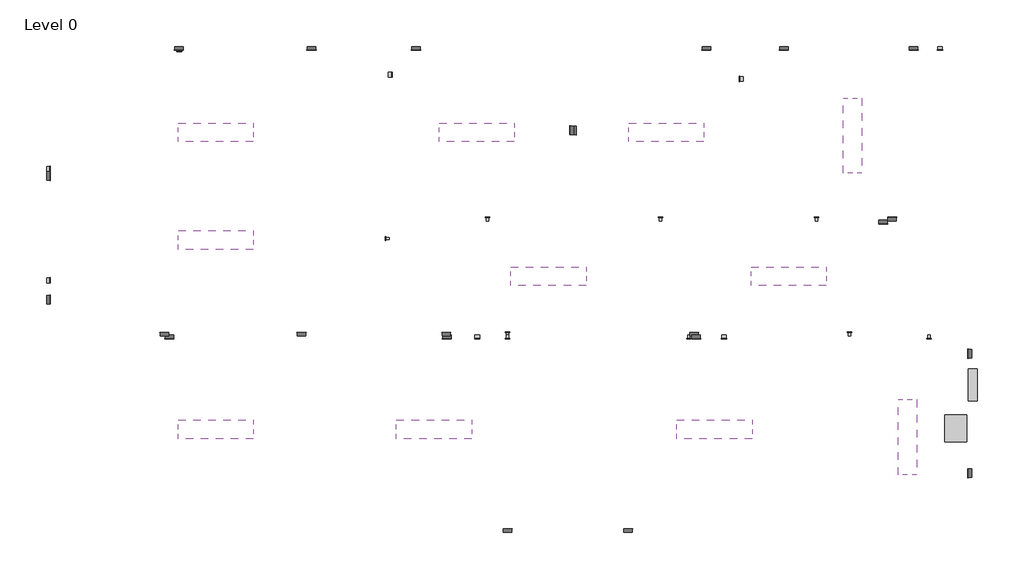
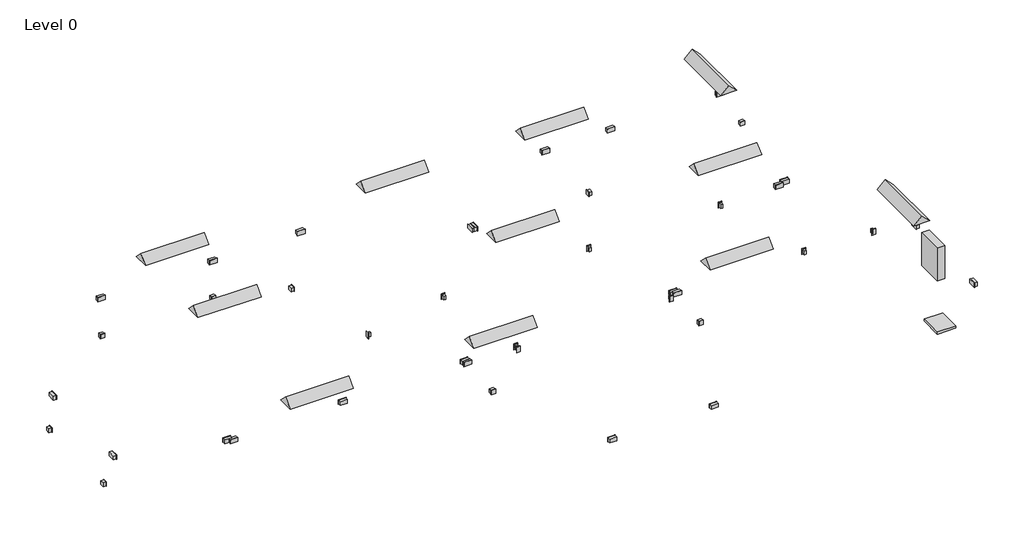
# One storey: 25 proxies, 11 light fixtures, 9 electric appliances, 9 switching devices.
"""IFC4 building model written with IfcOpenShell, lengths in millimetres."""

import ifcopenshell
import ifcopenshell.guid

model = None  # the IFC model being written
_history = None  # IfcOwnerHistory: only IFC2X3 demands one
_inside = {}  # id of a spatial element -> (the spatial element, [elements in it])
_under = {}  # id of a project, library or spatial element -> (it, [spatial elements below it])
_declared = {}  # id of a project -> (the project, [libraries it declares])
_typed = {}  # id of a type object -> (the type object, [elements of that type])
_made_of = {}  # id of a material, layer set ... -> (it, [elements and type objects made of it])


def new_model(schema):
    """Start an empty IFC model of exactly this schema.

    Asked for "IFC4X3", IfcOpenShell would pick the latest addendum, in which some entities
    have other attributes; the version numbers below select the first issue.
    IFC2X3 requires an IfcOwnerHistory on every rooted entity: one is made here for all.
    """
    global model, _history
    if schema == "IFC4X3":
        model = ifcopenshell.file(schema_version=(4, 3, 0, 0))
    else:
        model = ifcopenshell.file(schema=schema)
    _inside.clear()
    _under.clear()
    _declared.clear()
    _typed.clear()
    _made_of.clear()
    _history = None
    if model.schema == "IFC2X3":
        org = make("IfcOrganization", Name="unknown")
        user = make(
            "IfcPersonAndOrganization",
            ThePerson=make("IfcPerson", FamilyName="unknown"),
            TheOrganization=org,
        )
        app = make(
            "IfcApplication",
            ApplicationDeveloper=org,
            Version="unknown",
            ApplicationFullName="unknown",
            ApplicationIdentifier="unknown",
        )
        _history = make(
            "IfcOwnerHistory",
            OwningUser=user,
            OwningApplication=app,
            ChangeAction="ADDED",
            CreationDate=0,
        )
    return model


def make(cls, **values):
    """One entity of the class cls with the attributes given. An attribute that is None is left unset."""
    return model.create_entity(
        cls, **{name: value for name, value in values.items() if value is not None}
    )


def rooted(cls, **values):
    """An entity with a GlobalId (a new one), such as an element, a storey or a relation."""
    return make(cls, GlobalId=ifcopenshell.guid.new(), OwnerHistory=_history, **values)


def si_unit(unit_type, name, prefix=None):
    """IfcSIUnit, for example si_unit("LENGTHUNIT", "METRE", prefix="MILLI")."""
    return make("IfcSIUnit", UnitType=unit_type, Prefix=prefix, Name=name)


def assignment(units):
    """IfcUnitAssignment: the units of a project."""
    return None if units is None else make("IfcUnitAssignment", Units=units)


def point(xyz):
    """IfcCartesianPoint."""
    return None if xyz is None else make("IfcCartesianPoint", Coordinates=xyz)


def direction(xyz):
    """IfcDirection."""
    return None if xyz is None else make("IfcDirection", DirectionRatios=xyz)


def frame(location, z_axis=None, x_axis=None):
    """IfcAxis2Placement3D, a coordinate frame: its origin and axes. An axis left out is left unset."""
    return make(
        "IfcAxis2Placement3D",
        Location=point(location),
        Axis=direction(z_axis),
        RefDirection=direction(x_axis),
    )


def origin():
    """The frame at (0, 0, 0) with its axes left unset."""
    return frame((0.0, 0.0, 0.0))


def origin_with_axes():
    """The frame at (0, 0, 0) with the z axis (0, 0, 1) and the x axis (1, 0, 0) written out."""
    return frame((0.0, 0.0, 0.0), z_axis=(0.0, 0.0, 1.0), x_axis=(1.0, 0.0, 0.0))


def place(relative_to, where):
    """IfcLocalPlacement: puts the frame where relative to a parent placement (None: the world)."""
    return make(
        "IfcLocalPlacement", PlacementRelTo=relative_to, RelativePlacement=where
    )


def context(
    kind, dimensions, precision=None, world=None, true_north=None, identifier=None
):
    """IfcGeometricRepresentationContext, for example the 3D "Model" context."""
    return make(
        "IfcGeometricRepresentationContext",
        ContextIdentifier=identifier,
        ContextType=kind,
        CoordinateSpaceDimension=dimensions,
        Precision=precision,
        WorldCoordinateSystem=world,
        TrueNorth=true_north,
    )


def project(units=None, contexts=None):
    """IfcProject with its units and contexts."""
    return rooted(
        "IfcProject",
        Name="project",
        RepresentationContexts=contexts,
        UnitsInContext=assignment(units),
    )


def spatial(cls, under=None, at=None, **own):
    """A site, building, storey or space (cls), placed at a placement, below another one or the project."""
    s = rooted(cls, ObjectPlacement=at, **own)
    if under is not None:
        _under.setdefault(under.id(), (under, []))[1].append(s)
    return s


def polyline(points):
    """IfcPolyline through the points."""
    return make("IfcPolyline", Points=[point(p) for p in points])


def outline(outer, holes=None, kind="AREA"):
    """IfcArbitraryClosedProfileDef: a profile drawn as a closed curve; with holes, ...WithVoids."""
    if holes is None:
        return make("IfcArbitraryClosedProfileDef", ProfileType=kind, OuterCurve=outer)
    return make(
        "IfcArbitraryProfileDefWithVoids",
        ProfileType=kind,
        OuterCurve=outer,
        InnerCurves=holes,
    )


def extrude(swept, where, along, depth):
    """IfcExtrudedAreaSolid: the profile swept, set in the frame where, extruded along a direction by depth."""
    return make(
        "IfcExtrudedAreaSolid",
        SweptArea=swept,
        Position=where,
        ExtrudedDirection=direction(along),
        Depth=depth,
    )


def shape(context_of_items, identifier, shape_type, items):
    """IfcShapeRepresentation: the items that make up one representation, for example the "Body"."""
    return make(
        "IfcShapeRepresentation",
        ContextOfItems=context_of_items,
        RepresentationIdentifier=identifier,
        RepresentationType=shape_type,
        Items=items,
    )


def source(mapping_origin, context_of_items, identifier, shape_type, items):
    """IfcRepresentationMap: a shape defined once, which mapped items show again and again."""
    return make(
        "IfcRepresentationMap",
        MappingOrigin=mapping_origin,
        MappedRepresentation=shape(context_of_items, identifier, shape_type, items),
    )


def transform(
    local_origin,
    x_axis=None,
    y_axis=None,
    z_axis=None,
    scale=None,
    scale2=None,
    scale3=None,
    uniform=True,
):
    """IfcCartesianTransformationOperator3D, or its non-uniform kind. x_axis, y_axis, z_axis: its Axis1, 2, 3."""
    if uniform:
        return make(
            "IfcCartesianTransformationOperator3D",
            Axis1=direction(x_axis),
            Axis2=direction(y_axis),
            LocalOrigin=point(local_origin),
            Scale=scale,
            Axis3=direction(z_axis),
        )
    return make(
        "IfcCartesianTransformationOperator3DnonUniform",
        Axis1=direction(x_axis),
        Axis2=direction(y_axis),
        LocalOrigin=point(local_origin),
        Scale=scale,
        Axis3=direction(z_axis),
        Scale2=scale2,
        Scale3=scale3,
    )


def mapped(mapping_source, mapping_target):
    """IfcMappedItem: shows the shape of a source again, moved by a transform."""
    return make(
        "IfcMappedItem", MappingSource=mapping_source, MappingTarget=mapping_target
    )


def made_of(thing, what):
    """Note that an element or type object is made of a material, layer set ...; save() writes the relation."""
    if what is not None:
        _made_of.setdefault(what.id(), (what, []))[1].append(thing)
    return thing


def element(
    cls,
    number,
    at=None,
    inside=None,
    cuts=None,
    type_object=None,
    material=None,
    context=None,
    identifier="Body",
    shape_type=None,
    held_by="IfcProductDefinitionShape",
    body=None,
    shapes=None,
    **own,
):
    """One element of the class cls, such as IfcWall. Its Tag is "e" and its number.

    at: its placement. inside: the storey or other place that contains it. cuts: it is an
    opening in that element (IfcRelVoidsElement). A single representation is given by context,
    identifier, shape_type and body (its items); several are given by shapes. held_by: the class
    of the entity that holds the representations. save() writes the other relations.
    """
    e = rooted(cls, Tag="e%d" % number, ObjectPlacement=at, **own)
    if body is not None:
        shapes = [shape(context, identifier, shape_type, body)]
    if shapes is not None:
        e.Representation = make(held_by, Representations=shapes)
    if inside is not None:
        _inside.setdefault(inside.id(), (inside, []))[1].append(e)
    if cuts is not None:
        rooted(
            "IfcRelVoidsElement", RelatingBuildingElement=cuts, RelatedOpeningElement=e
        )
    if type_object is not None:
        _typed.setdefault(type_object.id(), (type_object, []))[1].append(e)
    return made_of(e, material)


def aggregate(whole, parts):
    """IfcRelAggregates: a whole, such as a stair, and the parts it consists of."""
    return rooted("IfcRelAggregates", RelatingObject=whole, RelatedObjects=parts)


def save(model, path):
    """Write the relations noted so far, then the file.

    IfcRelAggregates (storeys below a building ...), IfcRelContainedInSpatialStructure (elements
    in a storey), IfcRelDefinesByType, IfcRelAssociatesMaterial and IfcRelDeclares: one each for
    every whole, place, type object, material and project.
    """
    for whole, parts in _under.values():
        aggregate(whole, parts)
    for where, things in _inside.values():
        rooted(
            "IfcRelContainedInSpatialStructure",
            RelatedElements=things,
            RelatingStructure=where,
        )
    for kind, things in _typed.values():
        rooted("IfcRelDefinesByType", RelatedObjects=things, RelatingType=kind)
    for what, things in _made_of.values():
        rooted("IfcRelAssociatesMaterial", RelatedObjects=things, RelatingMaterial=what)
    for by, libraries in _declared.values():
        rooted("IfcRelDeclares", RelatingContext=by, RelatedDefinitions=libraries)
    model.write(path)


def ethernet_switch_5c8040eb(model_context):
    return source(origin(), model_context, "Body", "SweptSolid", [
        extrude(outline(polyline([(216.05, 174.5), (216.05, -174.5), (-216.05, -174.5), (-216.05, 174.5), (216.05, 174.5)])), origin_with_axes(), (0.0, 0.0, 1.0), 44.9),
    ])


def lighting_and_appliance_panelboard_400v_mlo_125_a_11cb7106(model_context):
    return source(origin(), model_context, "Body", "SweptSolid", [
        extrude(outline(polyline([(254.0, -660.4), (-254.0, -660.4), (-254.0, 0.0), (254.0, 0.0), (254.0, -660.4)])), frame((0.0, 0.0, -146.1), z_axis=(0.0, 0.0, 1.0), x_axis=(1.0, 0.0, 0.0)), (0.0, 0.0, 1.0), 146.1),
    ])


def twin_switched_socket_outlet_standard_0deee84c(model_context):
    return source(origin(), model_context, "Body", "SweptSolid", [
        extrude(outline(polyline([(67.5, 37.5), (67.5, -37.5), (-67.5, -37.5), (-67.5, 37.5), (67.5, 37.5)])), frame((0.0, 0.0, -53.975), z_axis=(0.0, 0.0, 1.0), x_axis=(1.0, 0.0, 0.0)), (0.0, 0.0, 1.0), 53.975),
        extrude(outline(polyline([(72.5, 42.5), (72.5, -42.5), (-72.5, -42.5), (-72.5, 42.5), (72.5, 42.5)])), origin_with_axes(), (0.0, 0.0, 1.0), 4.7625),
    ])


def data_outlet_plain_4a0886d3(model_context):
    return source(origin(), model_context, "Body", "SweptSolid", [
        extrude(outline(polyline([(42.5, 42.5), (42.5, -42.5), (-42.5, -42.5), (-42.5, 42.5), (42.5, 42.5)])), origin_with_axes(), (0.0, 0.0, 1.0), 4.7625),
        extrude(outline(polyline([(37.5, 37.5), (37.5, -37.5), (-37.5, -37.5), (-37.5, 37.5), (37.5, 37.5)])), frame((0.0, 0.0, -53.975), z_axis=(0.0, 0.0, 1.0), x_axis=(1.0, 0.0, 0.0)), (0.0, 0.0, 1.0), 53.975),
    ])


def emergency_recessed_lighting_fixture_300x1200_230_e46e8774(model_context):
    return source(origin(), model_context, "Body", "SweptSolid", [
        extrude(outline(polyline([(-300.0, 0.0), (0.0, 0.0), (-150.0, -150.0), (-300.0, 0.0)])), frame((0.0, 0.0, 0.0), z_axis=(1.0, 0.0, 0.0), x_axis=(0.0, 1.0, 0.0)), (0.0, 0.0, 1.0), 1200.0),
    ])


def lighting_switches_one_way_switch_9cbd35ee(model_context):
    return source(origin(), model_context, "Body", "SweptSolid", [
        extrude(outline(polyline([(35.0, -114.0), (-35.0, -114.0), (-35.0, 0.0), (35.0, 0.0), (35.0, -114.0)])), origin_with_axes(), (0.0, 0.0, 1.0), 5.0),
        extrude(outline(polyline([(19.0, -95.0), (-19.0, -95.0), (-19.0, -19.0), (19.0, -19.0), (19.0, -95.0)])), frame((0.0, 0.0, -54.0), z_axis=(0.0, 0.0, 1.0), x_axis=(1.0, 0.0, 0.0)), (0.0, 0.0, 1.0), 54.0),
    ])


model = new_model("IFC4")

# Units and contexts
model_context = context("Model", 3, world=origin())
ifc_project = project(units=[si_unit("LENGTHUNIT", "METRE", prefix="MILLI")], contexts=[model_context])

# Site, building, storey
site = spatial("IfcSite", under=ifc_project)
building = spatial("IfcBuilding", under=site)
storey = spatial("IfcBuildingStorey", under=building, Name="Level 0", Elevation=0.0)

# Proxies
placement = place(None, origin())
ethernet_switch_shape = ethernet_switch_5c8040eb(model_context)
element("IfcBuildingElementProxy", 1, Name="Ethernet Switch : NETGEAR 16 Port Gigabit Ethernet Plus Network Switch (GS116E)", ObjectType="Ethernet Switch : NETGEAR 16 Port Gigabit Ethernet Plus Network Switch (GS116E)", at=placement, inside=storey, context=model_context, shape_type="MappedRepresentation", body=[
    mapped(ethernet_switch_shape, transform((7132.6351684, -1921.8302068, 0.0), x_axis=(0.0, 1.0, 0.0), y_axis=(-1.0, 0.0, 0.0), z_axis=(0.0, 0.0, 1.0))),
])
lighting_and_appliance_panelboard_400v_mlo_125_a_shape = lighting_and_appliance_panelboard_400v_mlo_125_a_11cb7106(model_context)
element("IfcBuildingElementProxy", 2, Name="Lighting and Appliance Panelboard - 400V MLO : 125 A", ObjectType="Lighting and Appliance Panelboard - 400V MLO : 125 A", at=placement, inside=storey, context=model_context, shape_type="MappedRepresentation", body=[
    mapped(lighting_and_appliance_panelboard_400v_mlo_125_a_shape, transform((7333.0126521, -1228.5996446, 1200.0), x_axis=(0.0, -1.0, 0.0), y_axis=(0.0, 0.0, 1.0), z_axis=(-1.0, 0.0, 0.0))),
])
twin_switched_socket_outlet_standard_shape = twin_switched_socket_outlet_standard_0deee84c(model_context)
element("IfcBuildingElementProxy", 3, Name="Twin Switched Socket Outlet : Standard", ObjectType="Twin Switched Socket Outlet : Standard", at=placement, inside=storey, context=model_context, shape_type="MappedRepresentation", body=[
    mapped(twin_switched_socket_outlet_standard_shape, transform((7333.0126521, -731.9030192, 1200.0), x_axis=(0.0, -1.0, 0.0), y_axis=(0.0, 0.0, 1.0), z_axis=(-1.0, 0.0, 0.0))),
])
element("IfcBuildingElementProxy", 4, Name="Twin Switched Socket Outlet : Standard", ObjectType="Twin Switched Socket Outlet : Standard", at=placement, inside=storey, context=model_context, shape_type="MappedRepresentation", body=[
    mapped(twin_switched_socket_outlet_standard_shape, transform((7333.0126521, -2640.7763248, 1200.0), x_axis=(0.0, -1.0, 0.0), y_axis=(0.0, 0.0, 1.0), z_axis=(-1.0, 0.0, 0.0))),
])
element("IfcBuildingElementProxy", 5, Name="Twin Switched Socket Outlet : Standard", ObjectType="Twin Switched Socket Outlet : Standard", at=placement, inside=storey, context=model_context, shape_type="MappedRepresentation", body=[
    mapped(twin_switched_socket_outlet_standard_shape, transform((1908.0707872, -3530.9314954, 1200.0), x_axis=(-1.0, 0.0, 0.0), y_axis=(0.0, 0.0, 1.0), z_axis=(0.0, 1.0, 0.0))),
])
element("IfcBuildingElementProxy", 6, Name="Twin Switched Socket Outlet : Standard", ObjectType="Twin Switched Socket Outlet : Standard", at=placement, inside=storey, context=model_context, shape_type="MappedRepresentation", body=[
    mapped(twin_switched_socket_outlet_standard_shape, transform((2992.0804727, -488.4314954, 1200.0), x_axis=(1.0, 0.0, 0.0), y_axis=(0.0, 0.0, 1.0), z_axis=(0.0, -1.0, 0.0))),
])
element("IfcBuildingElementProxy", 7, Name="Twin Switched Socket Outlet : Standard", ObjectType="Twin Switched Socket Outlet : Standard", at=placement, inside=storey, context=model_context, shape_type="MappedRepresentation", body=[
    mapped(twin_switched_socket_outlet_standard_shape, transform((2958.20517, -393.4314954, 1200.0), x_axis=(-1.0, 0.0, 0.0), y_axis=(0.0, 0.0, 1.0), z_axis=(0.0, 1.0, 0.0))),
])
element("IfcBuildingElementProxy", 8, Name="Twin Switched Socket Outlet : Standard", ObjectType="Twin Switched Socket Outlet : Standard", at=placement, inside=storey, context=model_context, shape_type="MappedRepresentation", body=[
    mapped(twin_switched_socket_outlet_standard_shape, transform((-14.3526395, -3530.9314954, 1200.0), x_axis=(-1.0, 0.0, 0.0), y_axis=(0.0, 0.0, 1.0), z_axis=(0.0, 1.0, 0.0))),
])
element("IfcBuildingElementProxy", 9, Name="Twin Switched Socket Outlet : Standard", ObjectType="Twin Switched Socket Outlet : Standard", at=placement, inside=storey, context=model_context, shape_type="MappedRepresentation", body=[
    mapped(twin_switched_socket_outlet_standard_shape, transform((4391.3814995, 4119.0685046, 1200.0), x_axis=(1.0, 0.0, 0.0), y_axis=(0.0, 0.0, 1.0), z_axis=(0.0, -1.0, 0.0))),
])
element("IfcBuildingElementProxy", 10, Name="Twin Switched Socket Outlet : Standard", ObjectType="Twin Switched Socket Outlet : Standard", at=placement, inside=storey, context=model_context, shape_type="MappedRepresentation", body=[
    mapped(twin_switched_socket_outlet_standard_shape, transform((6460.720641, 4119.0685046, 1200.0), x_axis=(1.0, 0.0, 0.0), y_axis=(0.0, 0.0, 1.0), z_axis=(0.0, -1.0, 0.0))),
])
element("IfcBuildingElementProxy", 11, Name="Twin Switched Socket Outlet : Standard", ObjectType="Twin Switched Socket Outlet : Standard", at=placement, inside=storey, context=model_context, shape_type="MappedRepresentation", body=[
    mapped(twin_switched_socket_outlet_standard_shape, transform((3154.1965323, 4119.0685046, 1200.0), x_axis=(1.0, 0.0, 0.0), y_axis=(0.0, 0.0, 1.0), z_axis=(0.0, -1.0, 0.0))),
])
element("IfcBuildingElementProxy", 12, Name="Twin Switched Socket Outlet : Standard", ObjectType="Twin Switched Socket Outlet : Standard", at=placement, inside=storey, context=model_context, shape_type="MappedRepresentation", body=[
    mapped(twin_switched_socket_outlet_standard_shape, transform((-1477.8828984, 4119.0685046, 1200.0), x_axis=(1.0, 0.0, 0.0), y_axis=(0.0, 0.0, 1.0), z_axis=(0.0, -1.0, 0.0))),
])
element("IfcBuildingElementProxy", 13, Name="Twin Switched Socket Outlet : Standard", ObjectType="Twin Switched Socket Outlet : Standard", at=placement, inside=storey, context=model_context, shape_type="MappedRepresentation", body=[
    mapped(twin_switched_socket_outlet_standard_shape, transform((-994.5789843, -393.4314954, 1200.0), x_axis=(-1.0, 0.0, 0.0), y_axis=(0.0, 0.0, 1.0), z_axis=(0.0, 1.0, 0.0))),
])
element("IfcBuildingElementProxy", 14, Name="Twin Switched Socket Outlet : Standard", ObjectType="Twin Switched Socket Outlet : Standard", at=placement, inside=storey, context=model_context, shape_type="MappedRepresentation", body=[
    mapped(twin_switched_socket_outlet_standard_shape, transform((-983.8752261, -488.4314954, 1200.0), x_axis=(1.0, 0.0, 0.0), y_axis=(0.0, 0.0, 1.0), z_axis=(0.0, -1.0, 0.0))),
])
element("IfcBuildingElementProxy", 15, Name="Twin Switched Socket Outlet : Standard", ObjectType="Twin Switched Socket Outlet : Standard", at=placement, inside=storey, context=model_context, shape_type="MappedRepresentation", body=[
    mapped(twin_switched_socket_outlet_standard_shape, transform((-7316.9873479, 2106.2473929, 1200.0), x_axis=(0.0, 1.0, 0.0), y_axis=(0.0, 0.0, 1.0), z_axis=(1.0, 0.0, 0.0))),
])
element("IfcBuildingElementProxy", 16, Name="Twin Switched Socket Outlet : Standard", ObjectType="Twin Switched Socket Outlet : Standard", at=placement, inside=storey, context=model_context, shape_type="MappedRepresentation", body=[
    mapped(twin_switched_socket_outlet_standard_shape, transform((-7316.9873479, 133.0110122, 1200.0), x_axis=(0.0, 1.0, 0.0), y_axis=(0.0, 0.0, 1.0), z_axis=(1.0, 0.0, 0.0))),
])
element("IfcBuildingElementProxy", 17, Name="Twin Switched Socket Outlet : Standard", ObjectType="Twin Switched Socket Outlet : Standard", at=placement, inside=storey, context=model_context, shape_type="MappedRepresentation", body=[
    mapped(twin_switched_socket_outlet_standard_shape, transform((-5491.7999145, -393.4314954, 1200.0), x_axis=(-1.0, 0.0, 0.0), y_axis=(0.0, 0.0, 1.0), z_axis=(0.0, 1.0, 0.0))),
])
element("IfcBuildingElementProxy", 18, Name="Twin Switched Socket Outlet : Standard", ObjectType="Twin Switched Socket Outlet : Standard", at=placement, inside=storey, context=model_context, shape_type="MappedRepresentation", body=[
    mapped(twin_switched_socket_outlet_standard_shape, transform((-5410.6999104, -488.4314954, 1200.0), x_axis=(1.0, 0.0, 0.0), y_axis=(0.0, 0.0, 1.0), z_axis=(0.0, -1.0, 0.0))),
])
element("IfcBuildingElementProxy", 19, Name="Twin Switched Socket Outlet : Standard", ObjectType="Twin Switched Socket Outlet : Standard", at=placement, inside=storey, context=model_context, shape_type="MappedRepresentation", body=[
    mapped(twin_switched_socket_outlet_standard_shape, transform((-5260.1397144, 4119.0685046, 1200.0), x_axis=(1.0, 0.0, 0.0), y_axis=(0.0, 0.0, 1.0), z_axis=(0.0, -1.0, 0.0))),
])
element("IfcBuildingElementProxy", 20, Name="Twin Switched Socket Outlet : Standard", ObjectType="Twin Switched Socket Outlet : Standard", at=placement, inside=storey, context=model_context, shape_type="MappedRepresentation", body=[
    mapped(twin_switched_socket_outlet_standard_shape, transform((-3144.1513827, 4119.0685046, 1200.0), x_axis=(1.0, 0.0, 0.0), y_axis=(0.0, 0.0, 1.0), z_axis=(0.0, -1.0, 0.0))),
])
element("IfcBuildingElementProxy", 21, Name="Twin Switched Socket Outlet : Standard", ObjectType="Twin Switched Socket Outlet : Standard", at=placement, inside=storey, context=model_context, shape_type="MappedRepresentation", body=[
    mapped(twin_switched_socket_outlet_standard_shape, transform((-3304.0957389, -393.4314954, 1200.0), x_axis=(-1.0, 0.0, 0.0), y_axis=(0.0, 0.0, 1.0), z_axis=(0.0, 1.0, 0.0))),
])
element("IfcBuildingElementProxy", 22, Name="Twin Switched Socket Outlet : Standard", ObjectType="Twin Switched Socket Outlet : Standard", at=placement, inside=storey, context=model_context, shape_type="MappedRepresentation", body=[
    mapped(twin_switched_socket_outlet_standard_shape, transform((983.0126521, 2835.1015679, 1200.0), x_axis=(0.0, -1.0, 0.0), y_axis=(0.0, 0.0, 1.0), z_axis=(-1.0, 0.0, 0.0))),
])
element("IfcBuildingElementProxy", 23, Name="Twin Switched Socket Outlet : Standard", ObjectType="Twin Switched Socket Outlet : Standard", at=placement, inside=storey, context=model_context, shape_type="MappedRepresentation", body=[
    mapped(twin_switched_socket_outlet_standard_shape, transform((1078.0126521, 2831.4402609, 1200.0), x_axis=(0.0, 1.0, 0.0), y_axis=(0.0, 0.0, 1.0), z_axis=(1.0, 0.0, 0.0))),
])
element("IfcBuildingElementProxy", 24, Name="Twin Switched Socket Outlet : Standard", ObjectType="Twin Switched Socket Outlet : Standard", at=placement, inside=storey, context=model_context, shape_type="MappedRepresentation", body=[
    mapped(twin_switched_socket_outlet_standard_shape, transform((5974.113816, 1346.5685046, 1200.0), x_axis=(1.0, 0.0, 0.0), y_axis=(0.0, 0.0, 1.0), z_axis=(0.0, -1.0, 0.0))),
])
element("IfcBuildingElementProxy", 25, Name="Twin Switched Socket Outlet : Standard", ObjectType="Twin Switched Socket Outlet : Standard", at=placement, inside=storey, context=model_context, shape_type="MappedRepresentation", body=[
    mapped(twin_switched_socket_outlet_standard_shape, transform((6119.3761729, 1441.5685046, 1200.0), x_axis=(-1.0, 0.0, 0.0), y_axis=(0.0, 0.0, 1.0), z_axis=(0.0, 1.0, 0.0))),
])

# Electric appliances
data_outlet_plain_shape = data_outlet_plain_4a0886d3(model_context)
element("IfcElectricAppliance", 26, ObjectType="Data Outlet : Plain", at=placement, inside=storey, context=model_context, shape_type="MappedRepresentation", body=[
    mapped(data_outlet_plain_shape, transform((-3134.1176883, 4119.0685046, 460.0), x_axis=(1.0, 0.0, 0.0), y_axis=(0.0, 0.0, 1.0), z_axis=(0.0, -1.0, 0.0))),
])
element("IfcElectricAppliance", 27, ObjectType="Data Outlet : Plain", at=placement, inside=storey, context=model_context, shape_type="MappedRepresentation", body=[
    mapped(data_outlet_plain_shape, transform((-5252.8949019, 4094.0685046, 460.0), x_axis=(1.0, 0.0, 0.0), y_axis=(0.0, 0.0, 1.0), z_axis=(0.0, -1.0, 0.0))),
])
element("IfcElectricAppliance", 28, ObjectType="Data Outlet : Plain", at=placement, inside=storey, context=model_context, shape_type="MappedRepresentation", body=[
    mapped(data_outlet_plain_shape, transform((-7316.9873479, 2217.7762603, 460.0), x_axis=(0.0, 1.0, 0.0), y_axis=(0.0, 0.0, 1.0), z_axis=(1.0, 0.0, 0.0))),
])
element("IfcElectricAppliance", 29, ObjectType="Data Outlet : Plain", at=placement, inside=storey, context=model_context, shape_type="MappedRepresentation", body=[
    mapped(data_outlet_plain_shape, transform((-7316.9873479, 438.6837246, 460.0), x_axis=(0.0, 1.0, 0.0), y_axis=(0.0, 0.0, 1.0), z_axis=(1.0, 0.0, 0.0))),
])
element("IfcElectricAppliance", 30, ObjectType="Data Outlet : Plain", at=placement, inside=storey, context=model_context, shape_type="MappedRepresentation", body=[
    mapped(data_outlet_plain_shape, transform((-1864.4873479, 3722.2829913, 460.0), x_axis=(0.0, 1.0, 0.0), y_axis=(0.0, 0.0, 1.0), z_axis=(1.0, 0.0, 0.0))),
])
element("IfcElectricAppliance", 31, ObjectType="Data Outlet : Plain", at=placement, inside=storey, context=model_context, shape_type="MappedRepresentation", body=[
    mapped(data_outlet_plain_shape, transform((3685.5126521, 3655.8047081, 460.0), x_axis=(0.0, -1.0, 0.0), y_axis=(0.0, 0.0, 1.0), z_axis=(-1.0, 0.0, 0.0))),
])
element("IfcElectricAppliance", 32, ObjectType="Data Outlet : Plain", at=placement, inside=storey, context=model_context, shape_type="MappedRepresentation", body=[
    mapped(data_outlet_plain_shape, transform((6879.7438768, 4119.0685046, 460.0), x_axis=(1.0, 0.0, 0.0), y_axis=(0.0, 0.0, 1.0), z_axis=(0.0, -1.0, 0.0))),
])
element("IfcElectricAppliance", 33, ObjectType="Data Outlet : Plain", at=placement, inside=storey, context=model_context, shape_type="MappedRepresentation", body=[
    mapped(data_outlet_plain_shape, transform((3436.3374128, -488.4314954, 460.0), x_axis=(1.0, 0.0, 0.0), y_axis=(0.0, 0.0, 1.0), z_axis=(0.0, -1.0, 0.0))),
])
element("IfcElectricAppliance", 34, ObjectType="Data Outlet : Plain", at=placement, inside=storey, context=model_context, shape_type="MappedRepresentation", body=[
    mapped(data_outlet_plain_shape, transform((-500.838908, -488.4314954, 460.0), x_axis=(1.0, 0.0, 0.0), y_axis=(0.0, 0.0, 1.0), z_axis=(0.0, -1.0, 0.0))),
])

# Light fixtures
emergency_recessed_lighting_fixture_300x1200_230_shape = emergency_recessed_lighting_fixture_300x1200_230_e46e8774(model_context)
element("IfcLightFixture", 35, ObjectType="Emergency Recessed Lighting Fixture : 300x1200 - 230", at=placement, inside=storey, context=model_context, shape_type="MappedRepresentation", body=[
    mapped(emergency_recessed_lighting_fixture_300x1200_230_shape, transform((-5270.0307392, 932.4806964, 2750.0), x_axis=(1.0, 0.0, 0.0), y_axis=(0.0, -1.0, 0.0), z_axis=(0.0, 0.0, -1.0))),
])
element("IfcLightFixture", 36, ObjectType="Emergency Recessed Lighting Fixture : 300x1200 - 230", at=placement, inside=storey, context=model_context, shape_type="MappedRepresentation", body=[
    mapped(emergency_recessed_lighting_fixture_300x1200_230_shape, transform((-1789.2039186, -2089.1732245, 2750.0), x_axis=(1.0, 0.0, 0.0), y_axis=(0.0, -1.0, 0.0), z_axis=(0.0, 0.0, -1.0))),
])
element("IfcLightFixture", 37, ObjectType="Emergency Recessed Lighting Fixture : 300x1200 - 230", at=placement, inside=storey, context=model_context, shape_type="MappedRepresentation", body=[
    mapped(emergency_recessed_lighting_fixture_300x1200_230_shape, transform((35.7584033, 354.8115644, 2750.0), x_axis=(1.0, 0.0, 0.0), y_axis=(0.0, -1.0, 0.0), z_axis=(0.0, 0.0, -1.0))),
])
element("IfcLightFixture", 38, ObjectType="Plain Recessed Lighting Fixture : 300x1200 - 230", at=placement, inside=storey, context=model_context, shape_type="MappedRepresentation", body=[
    mapped(emergency_recessed_lighting_fixture_300x1200_230_shape, transform((-5270.0307392, 2652.1798309, 2750.0), x_axis=(1.0, 0.0, 0.0), y_axis=(0.0, -1.0, 0.0), z_axis=(0.0, 0.0, -1.0))),
])
element("IfcLightFixture", 39, ObjectType="Plain Recessed Lighting Fixture : 300x1200 - 230", at=placement, inside=storey, context=model_context, shape_type="MappedRepresentation", body=[
    mapped(emergency_recessed_lighting_fixture_300x1200_230_shape, transform((-5270.0307392, -2089.1732245, 2750.0), x_axis=(1.0, 0.0, 0.0), y_axis=(0.0, -1.0, 0.0), z_axis=(0.0, 0.0, -1.0))),
])
element("IfcLightFixture", 40, ObjectType="Plain Recessed Lighting Fixture : 300x1200 - 230", at=placement, inside=storey, context=model_context, shape_type="MappedRepresentation", body=[
    mapped(emergency_recessed_lighting_fixture_300x1200_230_shape, transform((2684.0288466, -2089.1732245, 2750.0), x_axis=(1.0, 0.0, 0.0), y_axis=(0.0, -1.0, 0.0), z_axis=(0.0, 0.0, -1.0))),
])
element("IfcLightFixture", 41, ObjectType="Plain Recessed Lighting Fixture : 300x1200 - 230", at=placement, inside=storey, context=model_context, shape_type="MappedRepresentation", body=[
    mapped(emergency_recessed_lighting_fixture_300x1200_230_shape, transform((-1107.8505835, 2652.1798309, 2750.0), x_axis=(1.0, 0.0, 0.0), y_axis=(0.0, -1.0, 0.0), z_axis=(0.0, 0.0, -1.0))),
])
element("IfcLightFixture", 42, ObjectType="Plain Recessed Lighting Fixture : 300x1200 - 230", at=placement, inside=storey, context=model_context, shape_type="MappedRepresentation", body=[
    mapped(emergency_recessed_lighting_fixture_300x1200_230_shape, transform((1913.8033373, 2652.1798309, 2750.0), x_axis=(1.0, 0.0, 0.0), y_axis=(0.0, -1.0, 0.0), z_axis=(0.0, 0.0, -1.0))),
])
element("IfcLightFixture", 43, ObjectType="Plain Recessed Lighting Fixture : 300x1200 - 230", at=placement, inside=storey, context=model_context, shape_type="MappedRepresentation", body=[
    mapped(emergency_recessed_lighting_fixture_300x1200_230_shape, transform((5336.1226433, 3350.5669994, 2750.0), x_axis=(0.0, -1.0, 0.0), y_axis=(-1.0, 0.0, 0.0), z_axis=(0.0, 0.0, -1.0))),
])
element("IfcLightFixture", 44, ObjectType="Plain Recessed Lighting Fixture : 300x1200 - 230", at=placement, inside=storey, context=model_context, shape_type="MappedRepresentation", body=[
    mapped(emergency_recessed_lighting_fixture_300x1200_230_shape, transform((3868.9911685, 354.8115644, 2750.0), x_axis=(1.0, 0.0, 0.0), y_axis=(0.0, -1.0, 0.0), z_axis=(0.0, 0.0, -1.0))),
])
element("IfcLightFixture", 45, ObjectType="Plain Recessed Lighting Fixture : 300x1200 - 230", at=placement, inside=storey, context=model_context, shape_type="MappedRepresentation", body=[
    mapped(emergency_recessed_lighting_fixture_300x1200_230_shape, transform((6212.25416, -1465.5868026, 2750.0), x_axis=(0.0, -1.0, 0.0), y_axis=(-1.0, 0.0, 0.0), z_axis=(0.0, 0.0, -1.0))),
])

# Switching devices
lighting_switches_one_way_switch_shape = lighting_switches_one_way_switch_9cbd35ee(model_context)
element("IfcSwitchingDevice", 46, ObjectType="Lighting Switches : One Way Switch", at=placement, inside=storey, context=model_context, shape_type="MappedRepresentation", body=[
    mapped(lighting_switches_one_way_switch_shape, transform((-1959.4873479, 1106.2790704, 1200.0), x_axis=(0.0, -1.0, 0.0), y_axis=(0.0, 0.0, 1.0), z_axis=(-1.0, 0.0, 0.0))),
])
element("IfcSwitchingDevice", 47, ObjectType="Lighting Switches : One Way Switch", at=placement, inside=storey, context=model_context, shape_type="MappedRepresentation", body=[
    mapped(lighting_switches_one_way_switch_shape, transform((-334.0931611, 1441.5685046, 1200.0), x_axis=(-1.0, 0.0, 0.0), y_axis=(0.0, 0.0, 1.0), z_axis=(0.0, 1.0, 0.0))),
])
element("IfcSwitchingDevice", 48, ObjectType="Lighting Switches : One Way Switch", at=placement, inside=storey, context=model_context, shape_type="MappedRepresentation", body=[
    mapped(lighting_switches_one_way_switch_shape, transform((2425.9086107, 1441.5685046, 1200.0), x_axis=(-1.0, 0.0, 0.0), y_axis=(0.0, 0.0, 1.0), z_axis=(0.0, 1.0, 0.0))),
])
element("IfcSwitchingDevice", 49, ObjectType="Lighting Switches : One Way Switch", at=placement, inside=storey, context=model_context, shape_type="MappedRepresentation", body=[
    mapped(lighting_switches_one_way_switch_shape, transform((4910.5243833, 1441.5685046, 1200.0), x_axis=(-1.0, 0.0, 0.0), y_axis=(0.0, 0.0, 1.0), z_axis=(0.0, 1.0, 0.0))),
])
element("IfcSwitchingDevice", 50, ObjectType="Lighting Switches : One Way Switch", at=placement, inside=storey, context=model_context, shape_type="MappedRepresentation", body=[
    mapped(lighting_switches_one_way_switch_shape, transform((6703.5460749, -488.4314954, 1200.0), x_axis=(1.0, 0.0, 0.0), y_axis=(0.0, 0.0, 1.0), z_axis=(0.0, -1.0, 0.0))),
])
element("IfcSwitchingDevice", 51, ObjectType="Lighting Switches : One Way Switch", at=placement, inside=storey, context=model_context, shape_type="MappedRepresentation", body=[
    mapped(lighting_switches_one_way_switch_shape, transform((2874.1640336, -488.4314954, 1200.0), x_axis=(1.0, 0.0, 0.0), y_axis=(0.0, 0.0, 1.0), z_axis=(0.0, -1.0, 0.0))),
])
element("IfcSwitchingDevice", 52, ObjectType="Lighting Switches : One Way Switch", at=placement, inside=storey, context=model_context, shape_type="MappedRepresentation", body=[
    mapped(lighting_switches_one_way_switch_shape, transform((-20.2852685, -488.4314954, 1200.0), x_axis=(1.0, 0.0, 0.0), y_axis=(0.0, 0.0, 1.0), z_axis=(0.0, -1.0, 0.0))),
])
element("IfcSwitchingDevice", 53, ObjectType="Lighting Switches : Two Way Switch", at=placement, inside=storey, context=model_context, shape_type="MappedRepresentation", body=[
    mapped(lighting_switches_one_way_switch_shape, transform((-18.1392133, -393.4314954, 1200.0), x_axis=(-1.0, 0.0, 0.0), y_axis=(0.0, 0.0, 1.0), z_axis=(0.0, 1.0, 0.0))),
])
element("IfcSwitchingDevice", 54, ObjectType="Lighting Switches : Two Way Switch", at=placement, inside=storey, context=model_context, shape_type="MappedRepresentation", body=[
    mapped(lighting_switches_one_way_switch_shape, transform((5435.784517, -393.4314954, 1200.0), x_axis=(-1.0, 0.0, 0.0), y_axis=(0.0, 0.0, 1.0), z_axis=(0.0, 1.0, 0.0))),
])

save(model, "model.ifc")

# Revit data of these elements
# Project information
#   Document_Suitability_Code = "A1"
#   Document_Suitability_Description = "Construction"
#   Project Issue Date = "Oct 2020"
#   Project Status = "Project Status"
#   Client Name = "Your Name Here"
#   Project Address = "Enter address here"
#   Project Name = "Revit MEP 01"
#   Project Number = "RMEP01"
# Type "Ethernet Switch : NETGEAR 16 Port Gigabit Ethernet Plus Network Switch (GS116E)"
#   Width = 432.1 mm
#   Height = 44.9 mm
#   Depth = 349 mm
#   built-in parameter 1140087 [instance default] = 1
#   Default Elevation = 0
# Type "Lighting and Appliance Panelboard - 400V MLO : 125 A"
#   built-in parameter 1140081 [instance default] = "Recessed"
#   built-in parameter 1140083 [instance default] = "Type 1"
#   Width = 508 mm
#   built-in parameter 1140082 [instance default] = 100 (stored number, unit not read)
#   built-in parameter 1140140 [instance default] = 1 (stored number, unit not read)
#   Height [instance default] = 660.4 mm
#   Depth = 146.1 mm
#   Default Elevation = 1200 mm
#   42 Circuit Height = 1117.6 mm
#   30 Circuit Height = 965.2 mm
#   18 Circuit Height = 660.4 mm
#   12 Circuit Height = 660.4 mm
#   built-in parameter 1140142 [instance default] = -1
#   built-in parameter 1140079 [instance default] = 12
#   built-in parameter 1155100 [instance default] = -1
#   Load Classification = Other
#   built-in parameter 1140087 [instance default] = element -7000014
# Type "Twin Switched Socket Outlet : Standard"
#   Label = "2"
#   Switch Voltage = 230 V
#   Load = 180 VA
#   Default Elevation = 1200 mm
#   Load Classification = Socket
#   Assembly Code = ""
# Type "Data Outlet : Plain"
#   Label = "D"
#   Default Elevation = 460 mm
#   Assembly Code = ""
# Type "Emergency Recessed Lighting Fixture : 300x1200 - 230"
#   Photometric Web File = "1x42A12.ies"
#   Width = 300 mm
#   Wattage = 64 W
#   built-in parameter 1150110 = 1 (stored number, unit not read)
#   built-in parameter 1150109 = 1 (stored number, unit not read)
#   built-in parameter 1150113 = 1 (stored number, unit not read)
#   Tilt Angle = -90.00°
#   Normal Voltage = 230 V
#   Lumens = 5699.84 lm
#   built-in parameter 1114217 = 0.88 (stored number, unit not read)
#   built-in parameter 1150115 = 1 (stored number, unit not read)
#   built-in parameter 1150105 = 453.579 (stored number, unit not read)
#   Length = 1200 mm
#   built-in parameter 1150112 = 1 (stored number, unit not read)
#   built-in parameter 1150114 = 1 (stored number, unit not read)
#   built-in parameter 1150107 = 4230 (stored number, unit not read)
#   built-in parameter 1150106 = 4.53579 (stored number, unit not read)
#   Emit from Rectangle Width = 300 mm
#   Emit from Rectangle Length = 1200 mm
#   Emergency Voltage = 230 V
#   Emergency Load = 32 VA
#   built-in parameter 1150104 = 8.27394 (stored number, unit not read)
#   Depth = 150 mm
#   Default Elevation = 2000 mm
#   built-in parameter 1114218 = 0.88 (stored number, unit not read)
#   built-in parameter 1150133 = 10 (stored number, unit not read)
#   Apparent Load = 64 VA
#   built-in parameter 1150134 = 8
#   built-in parameter 1150137 = 1
#   Color Filter = 16777215
#   built-in parameter 1140040 [instance default] = 1
#   Load Classification = Lighting - Dwelling Unit
#   Emit Shape Visible in Rendering = no
#   Dimming Lamp Color Temperature Shift = (empty or 0)
#   Assembly Code = ""
# Type "Plain Recessed Lighting Fixture : 300x1200 - 230"
#   Photometric Web File = "1x42A12.ies"
#   Width = 300 mm
#   Wattage = 64 W
#   built-in parameter 1150110 = 1 (stored number, unit not read)
#   built-in parameter 1150109 = 1 (stored number, unit not read)
#   built-in parameter 1150113 = 1 (stored number, unit not read)
#   Tilt Angle = -90.00°
#   Lumens = 5699.84 lm
#   built-in parameter 1114217 = 0.88 (stored number, unit not read)
#   built-in parameter 1150115 = 1 (stored number, unit not read)
#   built-in parameter 1150105 = 453.579 (stored number, unit not read)
#   Length = 1200 mm
#   built-in parameter 1150112 = 1 (stored number, unit not read)
#   built-in parameter 1150114 = 1 (stored number, unit not read)
#   built-in parameter 1150107 = 4230 (stored number, unit not read)
#   built-in parameter 1150106 = 4.53579 (stored number, unit not read)
#   Emit from Rectangle Width = 300 mm
#   Emit from Rectangle Length = 1200 mm
#   built-in parameter 1150104 = 8.27394 (stored number, unit not read)
#   Depth = 150 mm
#   Default Elevation = 2000 mm
#   Ballast Voltage = 230 V
#   built-in parameter 1114218 = 0.88 (stored number, unit not read)
#   built-in parameter 1150133 = 10 (stored number, unit not read)
#   Apparent Load = 64 VA
#   built-in parameter 1150134 = 8
#   built-in parameter 1150137 = 1
#   Color Filter = 16777215
#   built-in parameter 1140040 [instance default] = 1
#   Load Classification = Lighting - Dwelling Unit
#   Emit Shape Visible in Rendering = no
#   Dimming Lamp Color Temperature Shift = (empty or 0)
#   Assembly Code = ""
# Type "Lighting Switches : One Way Switch"
#   Label = ""
#   Width = 70 mm
#   Switch Voltage [instance default] = 230 V
#   Length = 114 mm
#   Height = 59 mm
#   Default Elevation = 1200 mm
#   Apparent Load = 0 VA
#   Visibility 7 = no
#   Visibility 6 = no
#   Visibility 5 = yes
#   Visibility 4 = no
#   Visibility 3 = no
#   Visibility 2 = no
#   Visibility 1 = no
#   Number of Poles = 1
#   Load Classification = Other
# Type "Lighting Switches : Two Way Switch"
#   Label = "2"
#   Width = 70 mm
#   Switch Voltage [instance default] = 230 V
#   Length = 114 mm
#   Height = 59 mm
#   Default Elevation = 1200 mm
#   Apparent Load = 0 VA
#   Visibility 7 = no
#   Visibility 6 = no
#   Visibility 5 = no
#   Visibility 4 = yes
#   Visibility 3 = no
#   Visibility 2 = no
#   Visibility 1 = no
#   Number of Poles = 1
#   Load Classification = Other
# Element 1 (IfcBuildingElementProxy, "Ethernet Switch : NETGEAR 16 Port Gigabit Ethernet Plus Network Switch (GS116E)")
#   Mark = "2"
#   Phase Created = New Construction
# Element 2 (IfcBuildingElementProxy, "Lighting and Appliance Panelboard - 400V MLO : 125 A")
#   built-in parameter 1140086 = "-"
#   built-in parameter 1140085 = "CT"
#   Panel Name = "Main Panel"
#   Mark = "1"
#   built-in parameter 1140081 = "Recessed"
#   built-in parameter 1140083 = "Type 1"
#   built-in parameter 1140082 = 100 (stored number, unit not read)
#   built-in parameter 1140140 = 1 (stored number, unit not read)
#   Height = 660.4 mm
#   built-in parameter 1140142 = -1
#   built-in parameter 1140079 = 12
#   built-in parameter 1155100 = -1
#   built-in parameter 1140064 = 230/400 Wye
#   built-in parameter 1140087 = element -7000010
#   Phase Created = New Construction
# Element 3 (IfcBuildingElementProxy, "Twin Switched Socket Outlet : Standard")
#   Mark = "1"
#   Phase Created = New Construction
# Element 4 (IfcBuildingElementProxy, "Twin Switched Socket Outlet : Standard")
#   Mark = "2"
#   Phase Created = New Construction
# Element 5 (IfcBuildingElementProxy, "Twin Switched Socket Outlet : Standard")
#   Mark = "3"
#   Phase Created = New Construction
# Element 6 (IfcBuildingElementProxy, "Twin Switched Socket Outlet : Standard")
#   Mark = "4"
#   Phase Created = New Construction
# Element 7 (IfcBuildingElementProxy, "Twin Switched Socket Outlet : Standard")
#   Mark = "5"
#   Phase Created = New Construction
# Element 8 (IfcBuildingElementProxy, "Twin Switched Socket Outlet : Standard")
#   Mark = "6"
#   Phase Created = New Construction
# Element 9 (IfcBuildingElementProxy, "Twin Switched Socket Outlet : Standard")
#   Mark = "9"
#   Phase Created = New Construction
# Element 10 (IfcBuildingElementProxy, "Twin Switched Socket Outlet : Standard")
#   Mark = "10"
#   Phase Created = New Construction
# Element 11 (IfcBuildingElementProxy, "Twin Switched Socket Outlet : Standard")
#   Mark = "11"
#   Phase Created = New Construction
# Element 12 (IfcBuildingElementProxy, "Twin Switched Socket Outlet : Standard")
#   Mark = "13"
#   Phase Created = New Construction
# Element 13 (IfcBuildingElementProxy, "Twin Switched Socket Outlet : Standard")
#   Mark = "14"
#   Phase Created = New Construction
# Element 14 (IfcBuildingElementProxy, "Twin Switched Socket Outlet : Standard")
#   Mark = "15"
#   Phase Created = New Construction
# Element 15 (IfcBuildingElementProxy, "Twin Switched Socket Outlet : Standard")
#   Mark = "16"
#   Phase Created = New Construction
# Element 16 (IfcBuildingElementProxy, "Twin Switched Socket Outlet : Standard")
#   Mark = "17"
#   Phase Created = New Construction
# Element 17 (IfcBuildingElementProxy, "Twin Switched Socket Outlet : Standard")
#   Mark = "18"
#   Phase Created = New Construction
# Element 18 (IfcBuildingElementProxy, "Twin Switched Socket Outlet : Standard")
#   Mark = "19"
#   Phase Created = New Construction
# Element 19 (IfcBuildingElementProxy, "Twin Switched Socket Outlet : Standard")
#   Mark = "20"
#   Phase Created = New Construction
# Element 20 (IfcBuildingElementProxy, "Twin Switched Socket Outlet : Standard")
#   Mark = "21"
#   Phase Created = New Construction
# Element 21 (IfcBuildingElementProxy, "Twin Switched Socket Outlet : Standard")
#   Mark = "22"
#   Phase Created = New Construction
# Element 22 (IfcBuildingElementProxy, "Twin Switched Socket Outlet : Standard")
#   Mark = "23"
#   Phase Created = New Construction
# Element 23 (IfcBuildingElementProxy, "Twin Switched Socket Outlet : Standard")
#   Mark = "24"
#   Phase Created = New Construction
# Element 24 (IfcBuildingElementProxy, "Twin Switched Socket Outlet : Standard")
#   Mark = "25"
#   Phase Created = New Construction
# Element 25 (IfcBuildingElementProxy, "Twin Switched Socket Outlet : Standard")
#   Mark = "26"
#   Phase Created = New Construction
# Element 26 (IfcElectricAppliance, "Data Outlet : Plain")
#   Mark = "1"
#   Phase Created = New Construction
# Element 27 (IfcElectricAppliance, "Data Outlet : Plain")
#   Mark = "2"
#   Phase Created = New Construction
# Element 28 (IfcElectricAppliance, "Data Outlet : Plain")
#   Mark = "3"
#   Phase Created = New Construction
# Element 29 (IfcElectricAppliance, "Data Outlet : Plain")
#   Mark = "4"
#   Phase Created = New Construction
# Element 30 (IfcElectricAppliance, "Data Outlet : Plain")
#   Mark = "5"
#   Phase Created = New Construction
# Element 31 (IfcElectricAppliance, "Data Outlet : Plain")
#   Mark = "6"
#   Phase Created = New Construction
# Element 32 (IfcElectricAppliance, "Data Outlet : Plain")
#   Mark = "7"
#   Phase Created = New Construction
# Element 33 (IfcElectricAppliance, "Data Outlet : Plain")
#   Mark = "8"
#   Phase Created = New Construction
# Element 34 (IfcElectricAppliance, "Data Outlet : Plain")
#   Mark = "9"
#   Phase Created = New Construction
# Element 35 (IfcLightFixture, "Emergency Recessed Lighting Fixture : 300x1200 - 230")
#   Mark = "2"
#   built-in parameter 1140040 = 1
#   Phase Created = New Construction
# Element 36 (IfcLightFixture, "Emergency Recessed Lighting Fixture : 300x1200 - 230")
#   Mark = "4"
#   built-in parameter 1140040 = 1
#   Phase Created = New Construction
# Element 37 (IfcLightFixture, "Emergency Recessed Lighting Fixture : 300x1200 - 230")
#   Mark = "9"
#   built-in parameter 1140040 = 1
#   Phase Created = New Construction
# Element 38 (IfcLightFixture, "Plain Recessed Lighting Fixture : 300x1200 - 230")
#   Mark = "1"
#   built-in parameter 1140040 = 1
#   Phase Created = New Construction
# Element 39 (IfcLightFixture, "Plain Recessed Lighting Fixture : 300x1200 - 230")
#   Mark = "3"
#   built-in parameter 1140040 = 1
#   Phase Created = New Construction
# Element 40 (IfcLightFixture, "Plain Recessed Lighting Fixture : 300x1200 - 230")
#   Mark = "5"
#   built-in parameter 1140040 = 1
#   Phase Created = New Construction
# Element 41 (IfcLightFixture, "Plain Recessed Lighting Fixture : 300x1200 - 230")
#   Mark = "6"
#   built-in parameter 1140040 = 1
#   Phase Created = New Construction
# Element 42 (IfcLightFixture, "Plain Recessed Lighting Fixture : 300x1200 - 230")
#   Mark = "7"
#   built-in parameter 1140040 = 1
#   Phase Created = New Construction
# Element 43 (IfcLightFixture, "Plain Recessed Lighting Fixture : 300x1200 - 230")
#   Mark = "8"
#   built-in parameter 1140040 = 1
#   Phase Created = New Construction
# Element 44 (IfcLightFixture, "Plain Recessed Lighting Fixture : 300x1200 - 230")
#   Mark = "10"
#   built-in parameter 1140040 = 1
#   Phase Created = New Construction
# Element 45 (IfcLightFixture, "Plain Recessed Lighting Fixture : 300x1200 - 230")
#   Mark = "11"
#   built-in parameter 1140040 = 1
#   Phase Created = New Construction
# Element 46 (IfcSwitchingDevice, "Lighting Switches : One Way Switch")
#   Switch ID = "MOffLS"
#   Mark = "1"
#   Switch Voltage = 230 V
#   Phase Created = New Construction
# Element 47 (IfcSwitchingDevice, "Lighting Switches : One Way Switch")
#   Switch ID = "MR1LS"
#   Mark = "2"
#   Switch Voltage = 230 V
#   Phase Created = New Construction
# Element 48 (IfcSwitchingDevice, "Lighting Switches : One Way Switch")
#   Switch ID = "MR2LS"
#   Mark = "3"
#   Switch Voltage = 230 V
#   Phase Created = New Construction
# Element 49 (IfcSwitchingDevice, "Lighting Switches : One Way Switch")
#   Switch ID = "MgrOffLS"
#   Mark = "4"
#   Switch Voltage = 230 V
#   Phase Created = New Construction
# Element 50 (IfcSwitchingDevice, "Lighting Switches : One Way Switch")
#   Switch ID = "ServLS"
#   Mark = "5"
#   Switch Voltage = 230 V
#   Phase Created = New Construction
# Element 51 (IfcSwitchingDevice, "Lighting Switches : One Way Switch")
#   Switch ID = "RecLS"
#   Mark = "6"
#   Switch Voltage = 230 V
#   Phase Created = New Construction
# Element 52 (IfcSwitchingDevice, "Lighting Switches : One Way Switch")
#   Switch ID = "PubLS"
#   Mark = "7"
#   Switch Voltage = 230 V
#   Phase Created = New Construction
# Element 53 (IfcSwitchingDevice, "Lighting Switches : Two Way Switch")
#   Switch ID = "CorLS1-1"
#   Mark = "8"
#   Switch Voltage = 230 V
#   Phase Created = New Construction
# Element 54 (IfcSwitchingDevice, "Lighting Switches : Two Way Switch")
#   Switch ID = "CorLS1-2"
#   Mark = "9"
#   Switch Voltage = 230 V
#   Phase Created = New Construction
